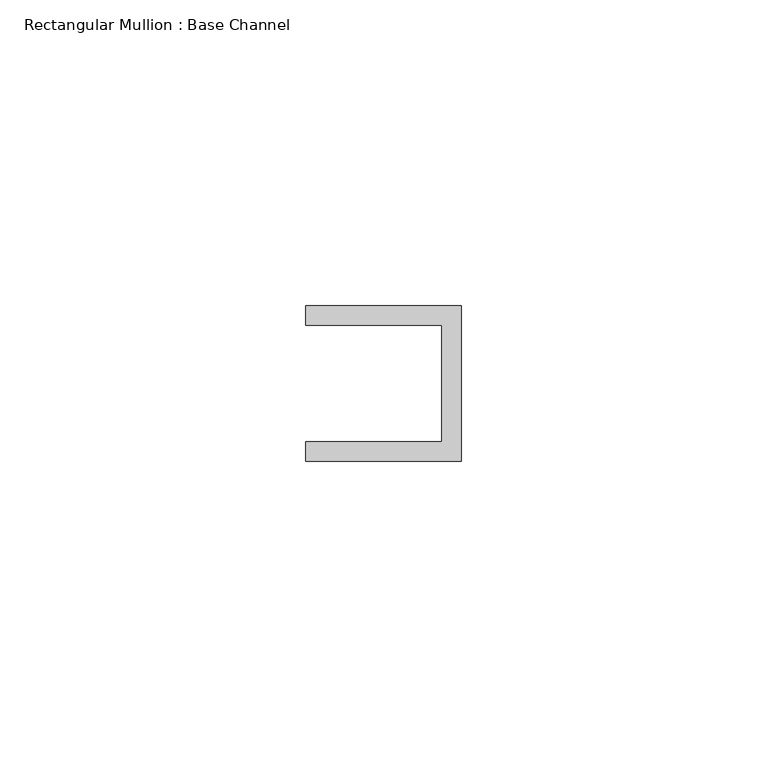
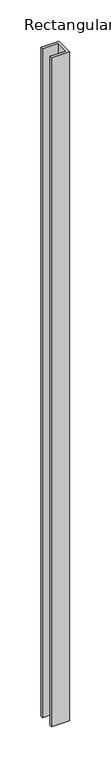
"""IFC4 building model written with IfcOpenShell, lengths in millimetres: member geometry, Rectangular Mullion : Base Channel."""

from ifc_helpers import new_model, si_unit, frame, origin, place, context, project, spatial, polyline, outline, extrude, source, transform, mapped, element, save


def rectangular_mullion_base_channel_029871b5(model_context):
    return source(origin(), model_context, "Body", "SweptSolid", [
        extrude(outline(polyline([(0.0, 12.7), (0.0, -12.7), (-25.4, -12.7), (-25.4, -9.525), (-3.175, -9.525), (-3.175, 9.525), (-25.4, 9.525), (-25.4, 12.7), (0.0, 12.7)])), frame((0.0, 0.0, -990.6), z_axis=(0.0, 0.0, 1.0), x_axis=(1.0, 0.0, 0.0)), (0.0, 0.0, 1.0), 990.6),
    ])


if __name__ == "__main__":
    model = new_model("IFC4")
    model_context = context("Model", 3, world=origin())
    ifc_project = project(units=[si_unit("LENGTHUNIT", "METRE", prefix="MILLI")], contexts=[model_context])
    site = spatial("IfcSite", under=ifc_project)
    building = spatial("IfcBuilding", under=site)
    placement = place(None, origin())
    rectangular_mullion_base_channel_shape = rectangular_mullion_base_channel_029871b5(model_context)
    element("IfcMember", 1, ObjectType="Rectangular Mullion : Base Channel", at=placement, inside=building, context=model_context, shape_type="MappedRepresentation", body=[
        mapped(rectangular_mullion_base_channel_shape, transform((0.0, 0.0, 0.0), x_axis=(1.0, 0.0, 0.0), y_axis=(0.0, 1.0, 0.0), z_axis=(0.0, 0.0, 1.0))),
    ])
    save(model, "model.ifc")

# Revit data of these elements
# Type "Rectangular Mullion : Base Channel"
#   built-in parameter 1007322 = 0.0833333 (stored number, unit not read)
#   built-in parameter 1007321 = 0.0416667 (stored number, unit not read)
#   built-in parameter 1007320 = -0.03125 (stored number, unit not read)
# Element 1 (IfcMember, "Rectangular Mullion : Base Channel")
#   Materials on its faces: "ALUM"
# Materials
#   "ALUM": class "Generic", colour RGB 157 157 157, transparency 0, Cost = 0
